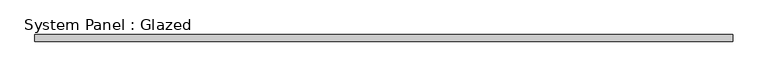
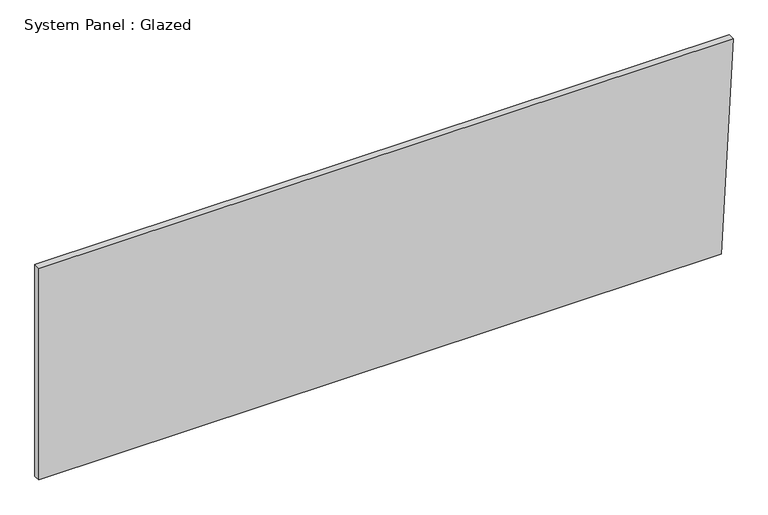
"""IFC4 building model written with IfcOpenShell, lengths in millimetres: plate geometry, System Panel : Glazed."""

import ifcopenshell
import ifcopenshell.guid

model = None  # the IFC model being written
_history = None  # IfcOwnerHistory: only IFC2X3 demands one
_inside = {}  # id of a spatial element -> (the spatial element, [elements in it])
_under = {}  # id of a project, library or spatial element -> (it, [spatial elements below it])
_declared = {}  # id of a project -> (the project, [libraries it declares])
_typed = {}  # id of a type object -> (the type object, [elements of that type])
_made_of = {}  # id of a material, layer set ... -> (it, [elements and type objects made of it])


def new_model(schema):
    """Start an empty IFC model of exactly this schema.

    Asked for "IFC4X3", IfcOpenShell would pick the latest addendum, in which some entities
    have other attributes; the version numbers below select the first issue.
    IFC2X3 requires an IfcOwnerHistory on every rooted entity: one is made here for all.
    """
    global model, _history
    if schema == "IFC4X3":
        model = ifcopenshell.file(schema_version=(4, 3, 0, 0))
    else:
        model = ifcopenshell.file(schema=schema)
    _inside.clear()
    _under.clear()
    _declared.clear()
    _typed.clear()
    _made_of.clear()
    _history = None
    if model.schema == "IFC2X3":
        org = make("IfcOrganization", Name="unknown")
        user = make(
            "IfcPersonAndOrganization",
            ThePerson=make("IfcPerson", FamilyName="unknown"),
            TheOrganization=org,
        )
        app = make(
            "IfcApplication",
            ApplicationDeveloper=org,
            Version="unknown",
            ApplicationFullName="unknown",
            ApplicationIdentifier="unknown",
        )
        _history = make(
            "IfcOwnerHistory",
            OwningUser=user,
            OwningApplication=app,
            ChangeAction="ADDED",
            CreationDate=0,
        )
    return model


def make(cls, **values):
    """One entity of the class cls with the attributes given. An attribute that is None is left unset."""
    return model.create_entity(
        cls, **{name: value for name, value in values.items() if value is not None}
    )


def rooted(cls, **values):
    """An entity with a GlobalId (a new one), such as an element, a storey or a relation."""
    return make(cls, GlobalId=ifcopenshell.guid.new(), OwnerHistory=_history, **values)


def si_unit(unit_type, name, prefix=None):
    """IfcSIUnit, for example si_unit("LENGTHUNIT", "METRE", prefix="MILLI")."""
    return make("IfcSIUnit", UnitType=unit_type, Prefix=prefix, Name=name)


def assignment(units):
    """IfcUnitAssignment: the units of a project."""
    return None if units is None else make("IfcUnitAssignment", Units=units)


def point(xyz):
    """IfcCartesianPoint."""
    return None if xyz is None else make("IfcCartesianPoint", Coordinates=xyz)


def direction(xyz):
    """IfcDirection."""
    return None if xyz is None else make("IfcDirection", DirectionRatios=xyz)


def frame(location, z_axis=None, x_axis=None):
    """IfcAxis2Placement3D, a coordinate frame: its origin and axes. An axis left out is left unset."""
    return make(
        "IfcAxis2Placement3D",
        Location=point(location),
        Axis=direction(z_axis),
        RefDirection=direction(x_axis),
    )


def origin():
    """The frame at (0, 0, 0) with its axes left unset."""
    return frame((0.0, 0.0, 0.0))


def place(relative_to, where):
    """IfcLocalPlacement: puts the frame where relative to a parent placement (None: the world)."""
    return make(
        "IfcLocalPlacement", PlacementRelTo=relative_to, RelativePlacement=where
    )


def context(
    kind, dimensions, precision=None, world=None, true_north=None, identifier=None
):
    """IfcGeometricRepresentationContext, for example the 3D "Model" context."""
    return make(
        "IfcGeometricRepresentationContext",
        ContextIdentifier=identifier,
        ContextType=kind,
        CoordinateSpaceDimension=dimensions,
        Precision=precision,
        WorldCoordinateSystem=world,
        TrueNorth=true_north,
    )


def project(units=None, contexts=None):
    """IfcProject with its units and contexts."""
    return rooted(
        "IfcProject",
        Name="project",
        RepresentationContexts=contexts,
        UnitsInContext=assignment(units),
    )


def spatial(cls, under=None, at=None, **own):
    """A site, building, storey or space (cls), placed at a placement, below another one or the project."""
    s = rooted(cls, ObjectPlacement=at, **own)
    if under is not None:
        _under.setdefault(under.id(), (under, []))[1].append(s)
    return s


def polyline(points):
    """IfcPolyline through the points."""
    return make("IfcPolyline", Points=[point(p) for p in points])


def outline(outer, holes=None, kind="AREA"):
    """IfcArbitraryClosedProfileDef: a profile drawn as a closed curve; with holes, ...WithVoids."""
    if holes is None:
        return make("IfcArbitraryClosedProfileDef", ProfileType=kind, OuterCurve=outer)
    return make(
        "IfcArbitraryProfileDefWithVoids",
        ProfileType=kind,
        OuterCurve=outer,
        InnerCurves=holes,
    )


def extrude(swept, where, along, depth):
    """IfcExtrudedAreaSolid: the profile swept, set in the frame where, extruded along a direction by depth."""
    return make(
        "IfcExtrudedAreaSolid",
        SweptArea=swept,
        Position=where,
        ExtrudedDirection=direction(along),
        Depth=depth,
    )


def shape(context_of_items, identifier, shape_type, items):
    """IfcShapeRepresentation: the items that make up one representation, for example the "Body"."""
    return make(
        "IfcShapeRepresentation",
        ContextOfItems=context_of_items,
        RepresentationIdentifier=identifier,
        RepresentationType=shape_type,
        Items=items,
    )


def source(mapping_origin, context_of_items, identifier, shape_type, items):
    """IfcRepresentationMap: a shape defined once, which mapped items show again and again."""
    return make(
        "IfcRepresentationMap",
        MappingOrigin=mapping_origin,
        MappedRepresentation=shape(context_of_items, identifier, shape_type, items),
    )


def transform(
    local_origin,
    x_axis=None,
    y_axis=None,
    z_axis=None,
    scale=None,
    scale2=None,
    scale3=None,
    uniform=True,
):
    """IfcCartesianTransformationOperator3D, or its non-uniform kind. x_axis, y_axis, z_axis: its Axis1, 2, 3."""
    if uniform:
        return make(
            "IfcCartesianTransformationOperator3D",
            Axis1=direction(x_axis),
            Axis2=direction(y_axis),
            LocalOrigin=point(local_origin),
            Scale=scale,
            Axis3=direction(z_axis),
        )
    return make(
        "IfcCartesianTransformationOperator3DnonUniform",
        Axis1=direction(x_axis),
        Axis2=direction(y_axis),
        LocalOrigin=point(local_origin),
        Scale=scale,
        Axis3=direction(z_axis),
        Scale2=scale2,
        Scale3=scale3,
    )


def mapped(mapping_source, mapping_target):
    """IfcMappedItem: shows the shape of a source again, moved by a transform."""
    return make(
        "IfcMappedItem", MappingSource=mapping_source, MappingTarget=mapping_target
    )


def made_of(thing, what):
    """Note that an element or type object is made of a material, layer set ...; save() writes the relation."""
    if what is not None:
        _made_of.setdefault(what.id(), (what, []))[1].append(thing)
    return thing


def element(
    cls,
    number,
    at=None,
    inside=None,
    cuts=None,
    type_object=None,
    material=None,
    context=None,
    identifier="Body",
    shape_type=None,
    held_by="IfcProductDefinitionShape",
    body=None,
    shapes=None,
    **own,
):
    """One element of the class cls, such as IfcWall. Its Tag is "e" and its number.

    at: its placement. inside: the storey or other place that contains it. cuts: it is an
    opening in that element (IfcRelVoidsElement). A single representation is given by context,
    identifier, shape_type and body (its items); several are given by shapes. held_by: the class
    of the entity that holds the representations. save() writes the other relations.
    """
    e = rooted(cls, Tag="e%d" % number, ObjectPlacement=at, **own)
    if body is not None:
        shapes = [shape(context, identifier, shape_type, body)]
    if shapes is not None:
        e.Representation = make(held_by, Representations=shapes)
    if inside is not None:
        _inside.setdefault(inside.id(), (inside, []))[1].append(e)
    if cuts is not None:
        rooted(
            "IfcRelVoidsElement", RelatingBuildingElement=cuts, RelatedOpeningElement=e
        )
    if type_object is not None:
        _typed.setdefault(type_object.id(), (type_object, []))[1].append(e)
    return made_of(e, material)


def aggregate(whole, parts):
    """IfcRelAggregates: a whole, such as a stair, and the parts it consists of."""
    return rooted("IfcRelAggregates", RelatingObject=whole, RelatedObjects=parts)


def save(model, path):
    """Write the relations noted so far, then the file.

    IfcRelAggregates (storeys below a building ...), IfcRelContainedInSpatialStructure (elements
    in a storey), IfcRelDefinesByType, IfcRelAssociatesMaterial and IfcRelDeclares: one each for
    every whole, place, type object, material and project.
    """
    for whole, parts in _under.values():
        aggregate(whole, parts)
    for where, things in _inside.values():
        rooted(
            "IfcRelContainedInSpatialStructure",
            RelatedElements=things,
            RelatingStructure=where,
        )
    for kind, things in _typed.values():
        rooted("IfcRelDefinesByType", RelatedObjects=things, RelatingType=kind)
    for what, things in _made_of.values():
        rooted("IfcRelAssociatesMaterial", RelatedObjects=things, RelatingMaterial=what)
    for by, libraries in _declared.values():
        rooted("IfcRelDeclares", RelatingContext=by, RelatedDefinitions=libraries)
    model.write(path)


def system_panel_glazed_ef221876(model_context):
    return source(origin(), model_context, "Body", "SweptSolid", [
        extrude(outline(polyline([(0.0, -1343.1943436), (0.0, 1297.8713084), (866.0018549, 1343.1943436), (866.0018549, -1343.1943436), (0.0, -1343.1943436)])), frame((0.0, -44.45, 0.0), z_axis=(0.0, 1.0, 0.0), x_axis=(0.0, 0.0, 1.0)), (0.0, 0.0, 1.0), 25.4),
    ])


if __name__ == "__main__":
    model = new_model("IFC4")
    model_context = context("Model", 3, world=origin())
    ifc_project = project(units=[si_unit("LENGTHUNIT", "METRE", prefix="MILLI")], contexts=[model_context])
    site = spatial("IfcSite", under=ifc_project)
    building = spatial("IfcBuilding", under=site)
    placement = place(None, origin())
    system_panel_glazed_shape = system_panel_glazed_ef221876(model_context)
    element("IfcPlate", 1, ObjectType="System Panel : Glazed", at=placement, inside=building, context=model_context, shape_type="MappedRepresentation", body=[
        mapped(system_panel_glazed_shape, transform((0.0, 0.0, 0.0), x_axis=(1.0, 0.0, 0.0), y_axis=(0.0, 1.0, 0.0), z_axis=(0.0, 0.0, 1.0))),
    ])
    save(model, "model.ifc")

# Revit data of these elements
# Type "System Panel : Glazed"
#   Construction Type Id = "GSP4R"
#   Analytic Construction = "1/8 in Pilkington single glazing"
#   Visual Light Transmittance = 0.9
#   Solar Heat Gain Coefficient = 0.86
#   Heat Transfer Coefficient (U) = 1.18115 BTU/(h·ft²·°F)
#   Define Thermal Properties by = 1
# Element 1 (IfcPlate, "System Panel : Glazed")
#   Materials on its faces: "Glass"
# Materials
#   "Glass": class "Glass", colour RGB 0 128 192, transparency 0.75, Description = "Soda Lime Glass", Cost = 0
